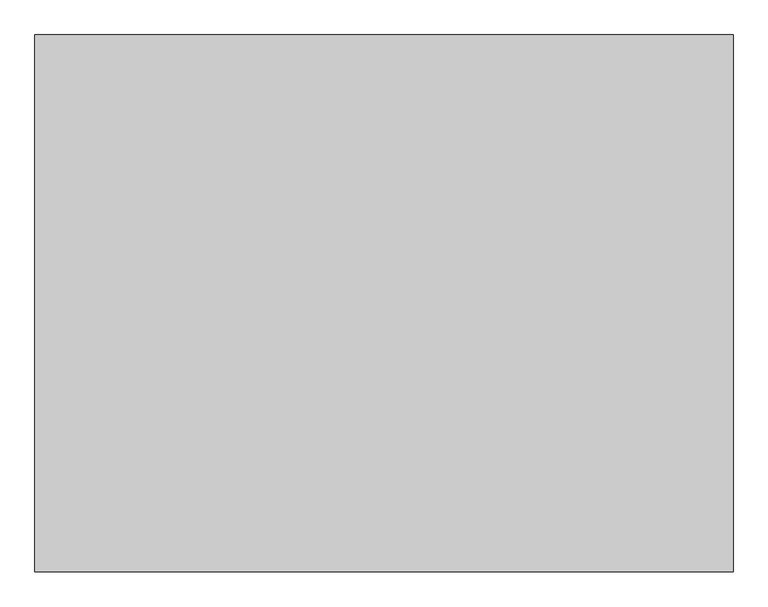
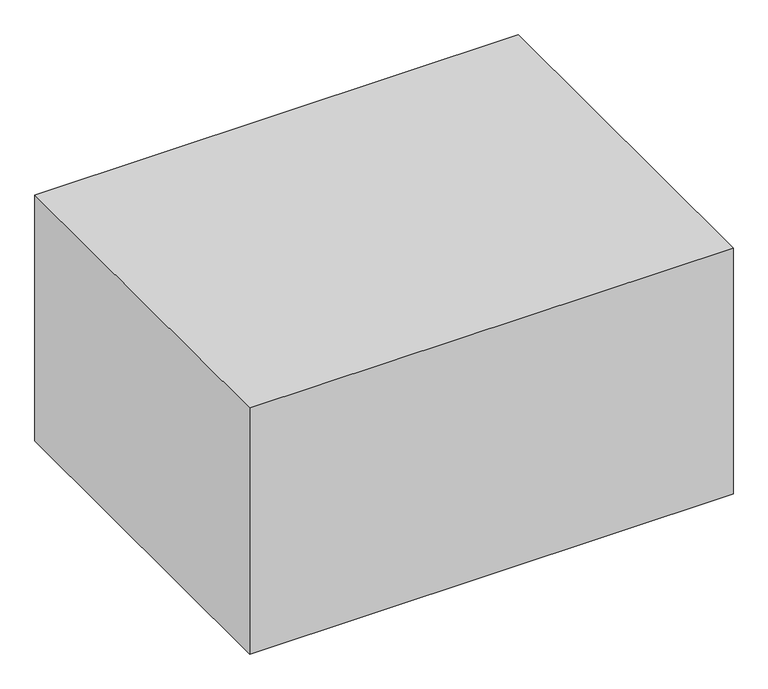
"""IFC4 building model written with IfcOpenShell, lengths in millimetres: proxy geometry, Space Planning Box_hec : Space Planning Box_hec."""

import ifcopenshell
import ifcopenshell.guid

model = None  # the IFC model being written
_history = None  # IfcOwnerHistory: only IFC2X3 demands one
_inside = {}  # id of a spatial element -> (the spatial element, [elements in it])
_under = {}  # id of a project, library or spatial element -> (it, [spatial elements below it])
_declared = {}  # id of a project -> (the project, [libraries it declares])
_typed = {}  # id of a type object -> (the type object, [elements of that type])
_made_of = {}  # id of a material, layer set ... -> (it, [elements and type objects made of it])


def new_model(schema):
    """Start an empty IFC model of exactly this schema.

    Asked for "IFC4X3", IfcOpenShell would pick the latest addendum, in which some entities
    have other attributes; the version numbers below select the first issue.
    IFC2X3 requires an IfcOwnerHistory on every rooted entity: one is made here for all.
    """
    global model, _history
    if schema == "IFC4X3":
        model = ifcopenshell.file(schema_version=(4, 3, 0, 0))
    else:
        model = ifcopenshell.file(schema=schema)
    _inside.clear()
    _under.clear()
    _declared.clear()
    _typed.clear()
    _made_of.clear()
    _history = None
    if model.schema == "IFC2X3":
        org = make("IfcOrganization", Name="unknown")
        user = make(
            "IfcPersonAndOrganization",
            ThePerson=make("IfcPerson", FamilyName="unknown"),
            TheOrganization=org,
        )
        app = make(
            "IfcApplication",
            ApplicationDeveloper=org,
            Version="unknown",
            ApplicationFullName="unknown",
            ApplicationIdentifier="unknown",
        )
        _history = make(
            "IfcOwnerHistory",
            OwningUser=user,
            OwningApplication=app,
            ChangeAction="ADDED",
            CreationDate=0,
        )
    return model


def make(cls, **values):
    """One entity of the class cls with the attributes given. An attribute that is None is left unset."""
    return model.create_entity(
        cls, **{name: value for name, value in values.items() if value is not None}
    )


def rooted(cls, **values):
    """An entity with a GlobalId (a new one), such as an element, a storey or a relation."""
    return make(cls, GlobalId=ifcopenshell.guid.new(), OwnerHistory=_history, **values)


def si_unit(unit_type, name, prefix=None):
    """IfcSIUnit, for example si_unit("LENGTHUNIT", "METRE", prefix="MILLI")."""
    return make("IfcSIUnit", UnitType=unit_type, Prefix=prefix, Name=name)


def assignment(units):
    """IfcUnitAssignment: the units of a project."""
    return None if units is None else make("IfcUnitAssignment", Units=units)


def point(xyz):
    """IfcCartesianPoint."""
    return None if xyz is None else make("IfcCartesianPoint", Coordinates=xyz)


def direction(xyz):
    """IfcDirection."""
    return None if xyz is None else make("IfcDirection", DirectionRatios=xyz)


def frame(location, z_axis=None, x_axis=None):
    """IfcAxis2Placement3D, a coordinate frame: its origin and axes. An axis left out is left unset."""
    return make(
        "IfcAxis2Placement3D",
        Location=point(location),
        Axis=direction(z_axis),
        RefDirection=direction(x_axis),
    )


def origin():
    """The frame at (0, 0, 0) with its axes left unset."""
    return frame((0.0, 0.0, 0.0))


def origin_with_axes():
    """The frame at (0, 0, 0) with the z axis (0, 0, 1) and the x axis (1, 0, 0) written out."""
    return frame((0.0, 0.0, 0.0), z_axis=(0.0, 0.0, 1.0), x_axis=(1.0, 0.0, 0.0))


def place(relative_to, where):
    """IfcLocalPlacement: puts the frame where relative to a parent placement (None: the world)."""
    return make(
        "IfcLocalPlacement", PlacementRelTo=relative_to, RelativePlacement=where
    )


def context(
    kind, dimensions, precision=None, world=None, true_north=None, identifier=None
):
    """IfcGeometricRepresentationContext, for example the 3D "Model" context."""
    return make(
        "IfcGeometricRepresentationContext",
        ContextIdentifier=identifier,
        ContextType=kind,
        CoordinateSpaceDimension=dimensions,
        Precision=precision,
        WorldCoordinateSystem=world,
        TrueNorth=true_north,
    )


def project(units=None, contexts=None):
    """IfcProject with its units and contexts."""
    return rooted(
        "IfcProject",
        Name="project",
        RepresentationContexts=contexts,
        UnitsInContext=assignment(units),
    )


def spatial(cls, under=None, at=None, **own):
    """A site, building, storey or space (cls), placed at a placement, below another one or the project."""
    s = rooted(cls, ObjectPlacement=at, **own)
    if under is not None:
        _under.setdefault(under.id(), (under, []))[1].append(s)
    return s


def polyline(points):
    """IfcPolyline through the points."""
    return make("IfcPolyline", Points=[point(p) for p in points])


def outline(outer, holes=None, kind="AREA"):
    """IfcArbitraryClosedProfileDef: a profile drawn as a closed curve; with holes, ...WithVoids."""
    if holes is None:
        return make("IfcArbitraryClosedProfileDef", ProfileType=kind, OuterCurve=outer)
    return make(
        "IfcArbitraryProfileDefWithVoids",
        ProfileType=kind,
        OuterCurve=outer,
        InnerCurves=holes,
    )


def extrude(swept, where, along, depth):
    """IfcExtrudedAreaSolid: the profile swept, set in the frame where, extruded along a direction by depth."""
    return make(
        "IfcExtrudedAreaSolid",
        SweptArea=swept,
        Position=where,
        ExtrudedDirection=direction(along),
        Depth=depth,
    )


def shape(context_of_items, identifier, shape_type, items):
    """IfcShapeRepresentation: the items that make up one representation, for example the "Body"."""
    return make(
        "IfcShapeRepresentation",
        ContextOfItems=context_of_items,
        RepresentationIdentifier=identifier,
        RepresentationType=shape_type,
        Items=items,
    )


def source(mapping_origin, context_of_items, identifier, shape_type, items):
    """IfcRepresentationMap: a shape defined once, which mapped items show again and again."""
    return make(
        "IfcRepresentationMap",
        MappingOrigin=mapping_origin,
        MappedRepresentation=shape(context_of_items, identifier, shape_type, items),
    )


def transform(
    local_origin,
    x_axis=None,
    y_axis=None,
    z_axis=None,
    scale=None,
    scale2=None,
    scale3=None,
    uniform=True,
):
    """IfcCartesianTransformationOperator3D, or its non-uniform kind. x_axis, y_axis, z_axis: its Axis1, 2, 3."""
    if uniform:
        return make(
            "IfcCartesianTransformationOperator3D",
            Axis1=direction(x_axis),
            Axis2=direction(y_axis),
            LocalOrigin=point(local_origin),
            Scale=scale,
            Axis3=direction(z_axis),
        )
    return make(
        "IfcCartesianTransformationOperator3DnonUniform",
        Axis1=direction(x_axis),
        Axis2=direction(y_axis),
        LocalOrigin=point(local_origin),
        Scale=scale,
        Axis3=direction(z_axis),
        Scale2=scale2,
        Scale3=scale3,
    )


def mapped(mapping_source, mapping_target):
    """IfcMappedItem: shows the shape of a source again, moved by a transform."""
    return make(
        "IfcMappedItem", MappingSource=mapping_source, MappingTarget=mapping_target
    )


def made_of(thing, what):
    """Note that an element or type object is made of a material, layer set ...; save() writes the relation."""
    if what is not None:
        _made_of.setdefault(what.id(), (what, []))[1].append(thing)
    return thing


def element(
    cls,
    number,
    at=None,
    inside=None,
    cuts=None,
    type_object=None,
    material=None,
    context=None,
    identifier="Body",
    shape_type=None,
    held_by="IfcProductDefinitionShape",
    body=None,
    shapes=None,
    **own,
):
    """One element of the class cls, such as IfcWall. Its Tag is "e" and its number.

    at: its placement. inside: the storey or other place that contains it. cuts: it is an
    opening in that element (IfcRelVoidsElement). A single representation is given by context,
    identifier, shape_type and body (its items); several are given by shapes. held_by: the class
    of the entity that holds the representations. save() writes the other relations.
    """
    e = rooted(cls, Tag="e%d" % number, ObjectPlacement=at, **own)
    if body is not None:
        shapes = [shape(context, identifier, shape_type, body)]
    if shapes is not None:
        e.Representation = make(held_by, Representations=shapes)
    if inside is not None:
        _inside.setdefault(inside.id(), (inside, []))[1].append(e)
    if cuts is not None:
        rooted(
            "IfcRelVoidsElement", RelatingBuildingElement=cuts, RelatedOpeningElement=e
        )
    if type_object is not None:
        _typed.setdefault(type_object.id(), (type_object, []))[1].append(e)
    return made_of(e, material)


def aggregate(whole, parts):
    """IfcRelAggregates: a whole, such as a stair, and the parts it consists of."""
    return rooted("IfcRelAggregates", RelatingObject=whole, RelatedObjects=parts)


def save(model, path):
    """Write the relations noted so far, then the file.

    IfcRelAggregates (storeys below a building ...), IfcRelContainedInSpatialStructure (elements
    in a storey), IfcRelDefinesByType, IfcRelAssociatesMaterial and IfcRelDeclares: one each for
    every whole, place, type object, material and project.
    """
    for whole, parts in _under.values():
        aggregate(whole, parts)
    for where, things in _inside.values():
        rooted(
            "IfcRelContainedInSpatialStructure",
            RelatedElements=things,
            RelatingStructure=where,
        )
    for kind, things in _typed.values():
        rooted("IfcRelDefinesByType", RelatedObjects=things, RelatingType=kind)
    for what, things in _made_of.values():
        rooted("IfcRelAssociatesMaterial", RelatedObjects=things, RelatingMaterial=what)
    for by, libraries in _declared.values():
        rooted("IfcRelDeclares", RelatingContext=by, RelatedDefinitions=libraries)
    model.write(path)


def generic_models_249c6621(model_context):
    return source(origin(), model_context, "Body", "SweptSolid", [
        extrude(outline(polyline([(3250.0, 2500.0), (3250.0, -2500.0), (-3250.0, -2500.0), (-3250.0, 2500.0), (3250.0, 2500.0)])), origin_with_axes(), (0.0, 0.0, 1.0), 3500.0),
    ])


if __name__ == "__main__":
    model = new_model("IFC4")
    model_context = context("Model", 3, world=origin())
    ifc_project = project(units=[si_unit("LENGTHUNIT", "METRE", prefix="MILLI")], contexts=[model_context])
    site = spatial("IfcSite", under=ifc_project)
    building = spatial("IfcBuilding", under=site)
    placement = place(None, origin())
    generic_models_shape = generic_models_249c6621(model_context)
    element("IfcBuildingElementProxy", 1, Name="Space Planning Box_hec : Space Planning Box_hec", ObjectType="Space Planning Box_hec : Space Planning Box_hec", at=placement, inside=building, context=model_context, shape_type="MappedRepresentation", body=[
        mapped(generic_models_shape, transform((0.0, 0.0, 0.0), x_axis=(1.0, 0.0, 0.0), y_axis=(0.0, 1.0, 0.0), z_axis=(0.0, 0.0, 1.0))),
    ])
    save(model, "model.ifc")

# Revit data of these elements
# Type "Space Planning Box_hec : Space Planning Box_hec"
#   Type Comments = "..."
#   Room Name [instance default] = "?"
#   Interior Finish [instance default] = ""
#   Exterior Finish [instance default] = ""
#   Department [instance default] = ""
#   Assembly Code = "..."
#   ceiling height [instance default] = 0
#   Width [instance default] = 1524 mm
#   Program Area [instance default] = 0.00 m²
#   Length [instance default] = 1524 mm
#   Height [instance default] = 1524 mm
#   Area [instance default] = 2.32258 m²
#   Fill Color [instance default] = Cyan
#   Default Elevation = 0
# Element 1 (IfcBuildingElementProxy, "Space Planning Box_hec : Space Planning Box_hec")
#   Room Name = "Office-1"
#   Exterior Finish = "RF1..N/A,,EW2..N/A..N/A"
#   Department = "AR"
#   Width = 6500 mm
#   Program Area = 32.50 m²
#   Length = 5000 mm
#   Height = 3500 mm
#   Area = 32.50 m²
#   Materials on its faces: "Cyan"
# Materials
#   "Cyan": class "Generic", colour RGB 0 255 255, transparency 0.2, Cost = 0
